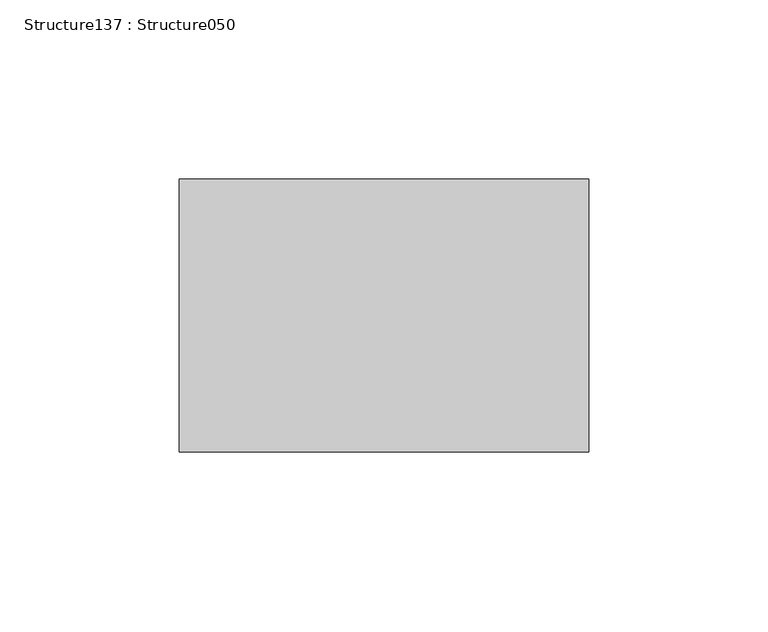
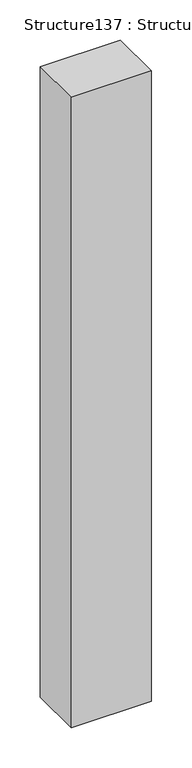
"""IFC4 building model written with IfcOpenShell, lengths in millimetres: proxy geometry, Structure137 : Structure050."""

from ifc_helpers import new_model, si_unit, frame, origin, place, context, project, spatial, polyline, outline, extrude, source, transform, mapped, element, save


def structure137_structure050_c5bf4f2a(model_context):
    return source(origin(), model_context, "Body", "SweptSolid", [
        extrude(outline(polyline([(-47526.4283589, 247945.1599557), (-47640.6644953, 247945.1599557), (-47640.6644953, 248021.3599557), (-47526.4283589, 248021.3599557), (-47526.4283589, 247945.1599557)])), frame((0.0, 0.0, 3528.5825142), z_axis=(0.0, 0.0, 1.0), x_axis=(1.0, 0.0, 0.0)), (0.0, 0.0, 1.0), 951.8594804),
    ])


if __name__ == "__main__":
    model = new_model("IFC4")
    model_context = context("Model", 3, world=origin())
    ifc_project = project(units=[si_unit("LENGTHUNIT", "METRE", prefix="MILLI")], contexts=[model_context])
    site = spatial("IfcSite", under=ifc_project)
    building = spatial("IfcBuilding", under=site)
    placement = place(None, origin())
    structure137_structure050_shape = structure137_structure050_c5bf4f2a(model_context)
    element("IfcBuildingElementProxy", 1, Name="Structure137 : Structure050", ObjectType="Structure137 : Structure050", at=placement, inside=building, context=model_context, shape_type="MappedRepresentation", body=[
        mapped(structure137_structure050_shape, transform((0.0, 0.0, 0.0), x_axis=(1.0, 0.0, 0.0), y_axis=(0.0, 1.0, 0.0), z_axis=(0.0, 0.0, 1.0))),
    ])
    save(model, "model.ifc")

# Revit data of these elements
# Type "Structure137 : Structure050"
#   NameOverride = "Structure050"
# Element 1 (IfcBuildingElementProxy, "Structure137 : Structure050")
#   Materials on its faces: "BRUSHED ALUM. LETTERING"
# Materials
#   "BRUSHED ALUM. LETTERING": class "Unassigned", colour RGB 169 181 186, transparency 0, Cost = 0
